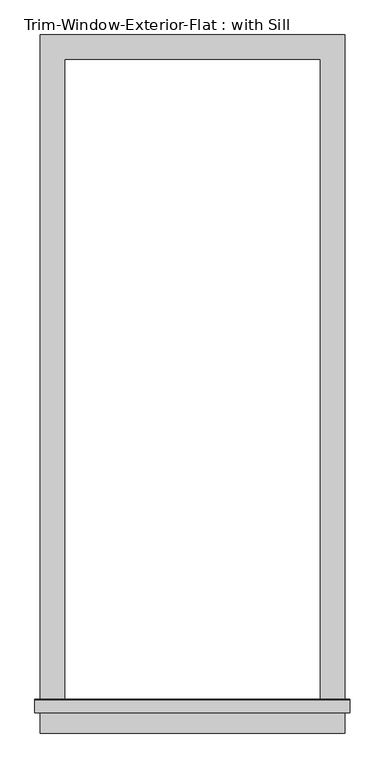
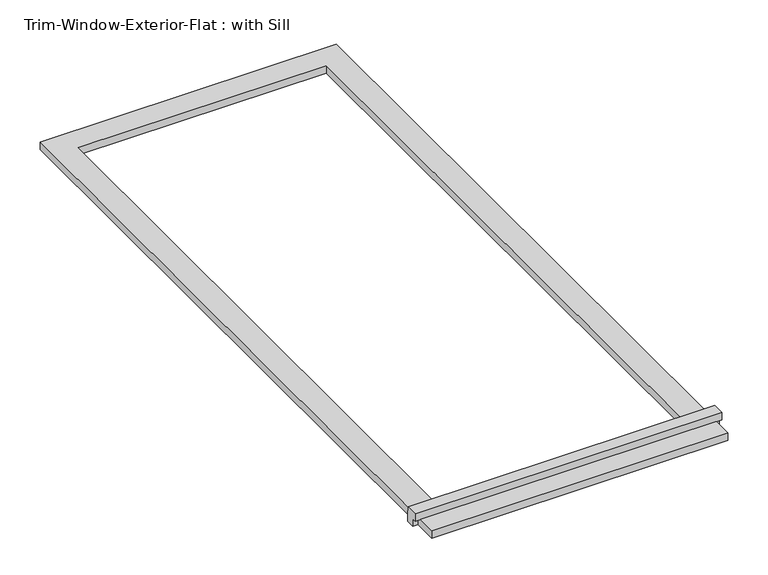
"""IFC4 building model written with IfcOpenShell, lengths in millimetres: proxy geometry, Trim-Window-Exterior-Flat : with Sill."""

from ifc_helpers import new_model, si_unit, frame, origin, origin_with_axes, place, context, project, spatial, polyline, outline, extrude, source, transform, mapped, element, save


def trim_window_exterior_flat_with_sill_2847f0e0(model_context):
    return source(origin(), model_context, "Body", "SweptSolid", [
        extrude(outline(polyline([(357.15, -1522.1823709), (357.15, -1579.3323709), (-357.15, -1579.3323709), (-357.15, -1522.1823709), (357.15, -1522.1823709)])), origin_with_axes(), (0.0, 0.0, 1.0), 19.05),
        extrude(outline(polyline([(-1531.75, 38.1), (-1502.4580645, 38.1), (-1500.0, 19.05), (-1500.0, 0.0), (-1522.1823709, 0.0), (-1522.1823709, 19.05), (-1531.75, 19.05), (-1531.75, 38.1)])), frame((-369.85, 0.0, 0.0), z_axis=(1.0, 0.0, 0.0), x_axis=(0.0, 1.0, 0.0)), (0.0, 0.0, 1.0), 739.7),
        extrude(outline(polyline([(-357.15, 57.15), (357.15, 57.15), (357.15, -1500.0), (300.0, -1500.0), (300.0, 0.0), (-300.0, 0.0), (-300.0, -1500.0), (-357.15, -1500.0), (-357.15, 57.15)])), origin_with_axes(), (0.0, 0.0, 1.0), 19.05),
    ])


if __name__ == "__main__":
    model = new_model("IFC4")
    model_context = context("Model", 3, world=origin())
    ifc_project = project(units=[si_unit("LENGTHUNIT", "METRE", prefix="MILLI")], contexts=[model_context])
    site = spatial("IfcSite", under=ifc_project)
    building = spatial("IfcBuilding", under=site)
    placement = place(None, origin())
    trim_window_exterior_flat_with_sill_shape = trim_window_exterior_flat_with_sill_2847f0e0(model_context)
    element("IfcBuildingElementProxy", 1, Name="Trim-Window-Exterior-Flat : with Sill", ObjectType="Trim-Window-Exterior-Flat : with Sill", at=placement, inside=building, context=model_context, shape_type="MappedRepresentation", body=[
        mapped(trim_window_exterior_flat_with_sill_shape, transform((0.0, 0.0, 0.0), x_axis=(1.0, 0.0, 0.0), y_axis=(0.0, 1.0, 0.0), z_axis=(0.0, 0.0, 1.0))),
    ])
    save(model, "model.ifc")

# Revit data of these elements
# Type "Trim-Window-Exterior-Flat : with Sill"
#   Trim Width = 5.715 cm
#   Trim Thickness_Picture Frame = 3.175 cm
#   Trim Thickness_with Sill = 1.905 cm
#   Sill Thickness = 3.175 cm
#   Opening Width [instance default] = 60.96 cm
#   Opening Height [instance default] = 91.44 cm
#   Default Elevation = 121.92 cm
#   Sill = yes
#   Picture Frame = no
#   Trim Material [instance default] = none
# Element 1 (IfcBuildingElementProxy, "Trim-Window-Exterior-Flat : with Sill")
#   Opening Width = 60 cm
#   Opening Height = 150 cm
#   Trim Material = Clad - White
#   Materials on its faces: "Clad - White"
# Materials
#   "Clad - White": class "Wood", colour RGB 242 242 238, transparency 0, Cost = 0
